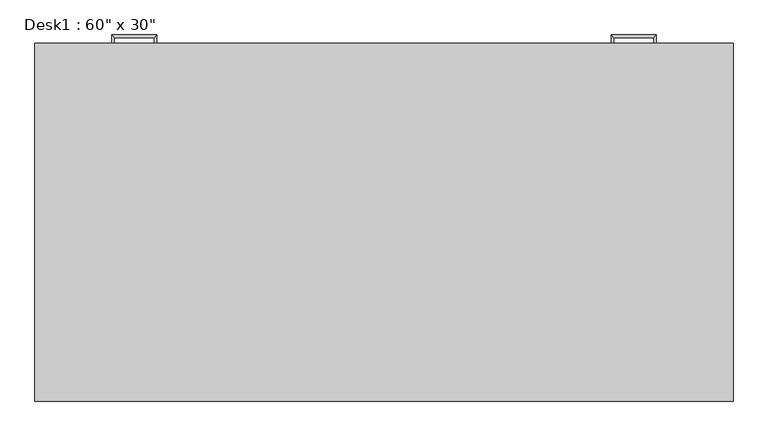
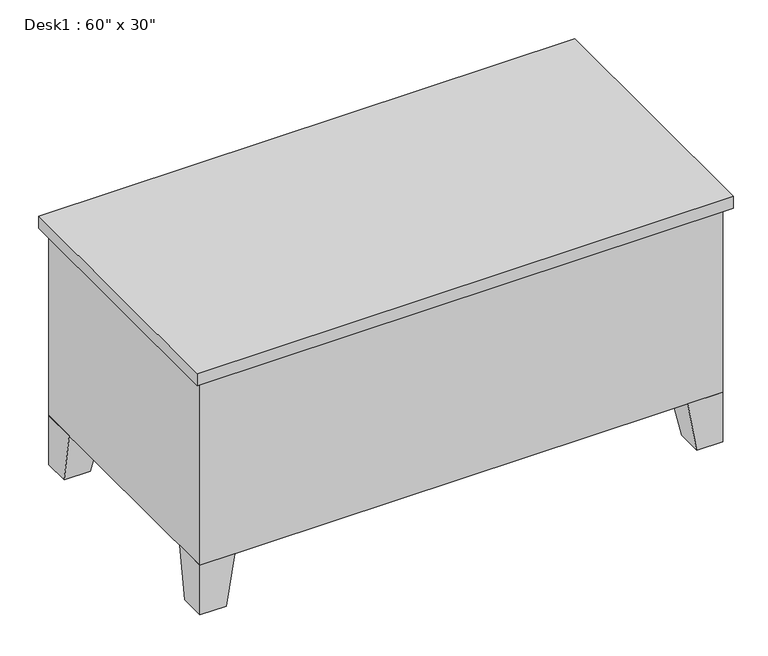
"""IFC4 building model written with IfcOpenShell, lengths in millimetres: furniture geometry."""

from ifc_helpers import new_model, si_unit, frame, origin, place, context, project, spatial, polyline, outline, extrude, faceted_brep, source, transform, mapped, element, save


def furniture_1092b3eb(model_context):
    return source(origin(), model_context, "Body", "SolidModel", [
        extrude(outline(polyline([(19.05, 0.0), (19.05, 12.7), (387.35, 12.7), (387.35, 0.0), (19.05, 0.0)])), frame((0.0, 0.0, 603.25), z_axis=(0.0, 0.0, 1.0), x_axis=(1.0, 0.0, 0.0)), (0.0, 0.0, 1.0), 101.6),
        extrude(outline(polyline([(19.05, 0.0), (19.05, 12.7), (387.35, 12.7), (387.35, 0.0), (19.05, 0.0)])), frame((0.0, 0.0, 171.45), z_axis=(0.0, 0.0, 1.0), x_axis=(1.0, 0.0, 0.0)), (0.0, 0.0, 1.0), 412.75),
        extrude(outline(polyline([(1136.65, 0.0), (1136.65, 12.7), (1504.95, 12.7), (1504.95, 0.0), (1136.65, 0.0)])), frame((0.0, 0.0, 603.25), z_axis=(0.0, 0.0, 1.0), x_axis=(1.0, 0.0, 0.0)), (0.0, 0.0, 1.0), 101.6),
        extrude(outline(polyline([(1136.65, 0.0), (1136.65, 12.7), (1504.95, 12.7), (1504.95, 0.0), (1136.65, 0.0)])), frame((0.0, 0.0, 171.45), z_axis=(0.0, 0.0, 1.0), x_axis=(1.0, 0.0, 0.0)), (0.0, 0.0, 1.0), 171.45),
        extrude(outline(polyline([(1136.65, 0.0), (1136.65, 12.7), (1504.95, 12.7), (1504.95, 0.0), (1136.65, 0.0)])), frame((0.0, 0.0, 482.6), z_axis=(0.0, 0.0, 1.0), x_axis=(1.0, 0.0, 0.0)), (0.0, 0.0, 1.0), 101.6),
        extrude(outline(polyline([(1136.65, 0.0), (1136.65, 12.7), (1504.95, 12.7), (1504.95, 0.0), (1136.65, 0.0)])), frame((0.0, 0.0, 361.95), z_axis=(0.0, 0.0, 1.0), x_axis=(1.0, 0.0, 0.0)), (0.0, 0.0, 1.0), 101.6),
        faceted_brep([(101.6, 0.0, 152.4), (0.0, 0.0, 152.4), (0.0, -101.6, 152.4), (101.6, -101.6, 152.4), (76.2, 0.0, 0.0), (76.2, -76.2, 0.0), (0.0, -76.2, 0.0), (0.0, 0.0, 0.0)], [[[0, 1, 2, 3]], [[4, 5, 6, 7]], [[4, 0, 3, 5]], [[5, 3, 2, 6]], [[6, 2, 1, 7]], [[7, 1, 0, 4]]]),
        faceted_brep([(101.6, -762.0, 152.4), (101.6, -660.4, 152.4), (0.0, -660.4, 152.4), (0.0, -762.0, 152.4), (76.2, -762.0, 0.0), (0.0, -762.0, 0.0), (0.0, -685.8, 0.0), (76.2, -685.8, 0.0)], [[[0, 1, 2, 3]], [[4, 5, 6, 7]], [[4, 0, 3, 5]], [[5, 3, 2, 6]], [[6, 2, 1, 7]], [[7, 1, 0, 4]]]),
        faceted_brep([(1422.4, -762.0, 152.4), (1524.0, -762.0, 152.4), (1524.0, -660.4, 152.4), (1422.4, -660.4, 152.4), (1447.8, -762.0, 0.0), (1447.8, -685.8, 0.0), (1524.0, -685.8, 0.0), (1524.0, -762.0, 0.0)], [[[0, 1, 2, 3]], [[4, 5, 6, 7]], [[4, 0, 3, 5]], [[5, 3, 2, 6]], [[6, 2, 1, 7]], [[7, 1, 0, 4]]]),
        faceted_brep([(1422.4, 0.0, 152.4), (1422.4, -101.6, 152.4), (1524.0, -101.6, 152.4), (1524.0, 0.0, 152.4), (1447.8, 0.0, 0.0), (1524.0, 0.0, 0.0), (1524.0, -76.2, 0.0), (1447.8, -76.2, 0.0)], [[[0, 1, 2, 3]], [[4, 5, 6, 7]], [[4, 0, 3, 5]], [[5, 3, 2, 6]], [[6, 2, 1, 7]], [[7, 1, 0, 4]]]),
        extrude(outline(polyline([(-19.05, 19.05), (1543.05, 19.05), (1543.05, -781.05), (-19.05, -781.05), (-19.05, 19.05)])), frame((0.0, 0.0, 723.9), z_axis=(0.0, 0.0, 1.0), x_axis=(1.0, 0.0, 0.0)), (0.0, 0.0, 1.0), 38.1),
        extrude(outline(polyline([(1117.6, 0.0), (1524.0, 0.0), (1524.0, -762.0), (0.0, -762.0), (0.0, 0.0), (406.4, 0.0), (406.4, -635.0), (1117.6, -635.0), (1117.6, 0.0)])), frame((0.0, 0.0, 152.4), z_axis=(0.0, 0.0, 1.0), x_axis=(1.0, 0.0, 0.0)), (0.0, 0.0, 1.0), 571.5),
        faceted_brep([(158.75, 12.7, 546.1), (152.4, 12.7, 546.1), (152.4, 12.7, 533.4), (158.75, 12.7, 533.4), (158.75, 31.75, 533.4), (158.75, 31.75, 546.1), (152.4, 38.1, 533.4), (152.4, 38.1, 546.1), (247.65, 31.75, 533.4), (247.65, 31.75, 546.1), (254.0, 38.1, 533.4), (254.0, 38.1, 546.1), (247.65, 12.7, 546.1), (247.65, 12.7, 533.4), (254.0, 12.7, 533.4), (254.0, 12.7, 546.1)], [[[0, 1, 2, 3]], [[3, 4, 5, 0]], [[2, 6, 4, 3]], [[1, 7, 6, 2]], [[0, 5, 7, 1]], [[4, 8, 9, 5]], [[6, 10, 8, 4]], [[7, 11, 10, 6]], [[5, 9, 11, 7]], [[12, 13, 14, 15]], [[8, 13, 12, 9]], [[10, 14, 13, 8]], [[11, 15, 14, 10]], [[9, 12, 15, 11]]]),
        faceted_brep([(158.75, 12.7, 666.75), (152.4, 12.7, 666.75), (152.4, 12.7, 654.05), (158.75, 12.7, 654.05), (158.75, 31.75, 654.05), (158.75, 31.75, 666.75), (152.4, 38.1, 654.05), (152.4, 38.1, 666.75), (247.65, 31.75, 654.05), (247.65, 31.75, 666.75), (254.0, 38.1, 654.05), (254.0, 38.1, 666.75), (247.65, 12.7, 666.75), (247.65, 12.7, 654.05), (254.0, 12.7, 654.05), (254.0, 12.7, 666.75)], [[[0, 1, 2, 3]], [[3, 4, 5, 0]], [[2, 6, 4, 3]], [[1, 7, 6, 2]], [[0, 5, 7, 1]], [[4, 8, 9, 5]], [[6, 10, 8, 4]], [[7, 11, 10, 6]], [[5, 9, 11, 7]], [[12, 13, 14, 15]], [[8, 13, 12, 9]], [[10, 14, 13, 8]], [[11, 15, 14, 10]], [[9, 12, 15, 11]]]),
        faceted_brep([(1365.25, 12.7, 304.8), (1365.25, 12.7, 292.1), (1371.6, 12.7, 292.1), (1371.6, 12.7, 304.8), (1371.6, 38.1, 304.8), (1365.25, 31.75, 304.8), (1371.6, 38.1, 292.1), (1365.25, 31.75, 292.1), (1270.0, 38.1, 304.8), (1276.35, 31.75, 304.8), (1270.0, 38.1, 292.1), (1276.35, 31.75, 292.1), (1276.35, 12.7, 304.8), (1270.0, 12.7, 304.8), (1270.0, 12.7, 292.1), (1276.35, 12.7, 292.1)], [[[0, 1, 2, 3]], [[3, 4, 5, 0]], [[2, 6, 4, 3]], [[1, 7, 6, 2]], [[0, 5, 7, 1]], [[4, 8, 9, 5]], [[6, 10, 8, 4]], [[7, 11, 10, 6]], [[5, 9, 11, 7]], [[12, 13, 14, 15]], [[8, 13, 12, 9]], [[10, 14, 13, 8]], [[11, 15, 14, 10]], [[9, 12, 15, 11]]]),
        faceted_brep([(1365.25, 12.7, 425.45), (1365.25, 12.7, 412.75), (1371.6, 12.7, 412.75), (1371.6, 12.7, 425.45), (1371.6, 38.1, 425.45), (1365.25, 31.75, 425.45), (1371.6, 38.1, 412.75), (1365.25, 31.75, 412.75), (1270.0, 38.1, 425.45), (1276.35, 31.75, 425.45), (1270.0, 38.1, 412.75), (1276.35, 31.75, 412.75), (1276.35, 12.7, 425.45), (1270.0, 12.7, 425.45), (1270.0, 12.7, 412.75), (1276.35, 12.7, 412.75)], [[[0, 1, 2, 3]], [[3, 4, 5, 0]], [[2, 6, 4, 3]], [[1, 7, 6, 2]], [[0, 5, 7, 1]], [[4, 8, 9, 5]], [[6, 10, 8, 4]], [[7, 11, 10, 6]], [[5, 9, 11, 7]], [[12, 13, 14, 15]], [[8, 13, 12, 9]], [[10, 14, 13, 8]], [[11, 15, 14, 10]], [[9, 12, 15, 11]]]),
        faceted_brep([(1365.25, 12.7, 546.1), (1365.25, 12.7, 533.4), (1371.6, 12.7, 533.4), (1371.6, 12.7, 546.1), (1371.6, 38.1, 546.1), (1365.25, 31.75, 546.1), (1371.6, 38.1, 533.4), (1365.25, 31.75, 533.4), (1270.0, 38.1, 546.1), (1276.35, 31.75, 546.1), (1270.0, 38.1, 533.4), (1276.35, 31.75, 533.4), (1276.35, 12.7, 546.1), (1270.0, 12.7, 546.1), (1270.0, 12.7, 533.4), (1276.35, 12.7, 533.4)], [[[0, 1, 2, 3]], [[3, 4, 5, 0]], [[2, 6, 4, 3]], [[1, 7, 6, 2]], [[0, 5, 7, 1]], [[4, 8, 9, 5]], [[6, 10, 8, 4]], [[7, 11, 10, 6]], [[5, 9, 11, 7]], [[12, 13, 14, 15]], [[8, 13, 12, 9]], [[10, 14, 13, 8]], [[11, 15, 14, 10]], [[9, 12, 15, 11]]]),
        faceted_brep([(1365.25, 12.7, 666.75), (1365.25, 12.7, 654.05), (1371.6, 12.7, 654.05), (1371.6, 12.7, 666.75), (1371.6, 38.1, 666.75), (1365.25, 31.75, 666.75), (1371.6, 38.1, 654.05), (1365.25, 31.75, 654.05), (1270.0, 38.1, 666.75), (1276.35, 31.75, 666.75), (1270.0, 38.1, 654.05), (1276.35, 31.75, 654.05), (1276.35, 12.7, 666.75), (1270.0, 12.7, 666.75), (1270.0, 12.7, 654.05), (1276.35, 12.7, 654.05)], [[[0, 1, 2, 3]], [[3, 4, 5, 0]], [[2, 6, 4, 3]], [[1, 7, 6, 2]], [[0, 5, 7, 1]], [[4, 8, 9, 5]], [[6, 10, 8, 4]], [[7, 11, 10, 6]], [[5, 9, 11, 7]], [[12, 13, 14, 15]], [[8, 13, 12, 9]], [[10, 14, 13, 8]], [[11, 15, 14, 10]], [[9, 12, 15, 11]]]),
    ])


if __name__ == "__main__":
    model = new_model("IFC4")
    model_context = context("Model", 3, world=origin())
    ifc_project = project(units=[si_unit("LENGTHUNIT", "METRE", prefix="MILLI")], contexts=[model_context])
    site = spatial("IfcSite", under=ifc_project)
    building = spatial("IfcBuilding", under=site)
    placement = place(None, origin())
    furniture_shape = furniture_1092b3eb(model_context)
    element("IfcFurniture", 1, ObjectType="Desk1 : 60\" x 30\"", at=placement, inside=building, context=model_context, shape_type="MappedRepresentation", body=[
        mapped(furniture_shape, transform((0.0, 0.0, 0.0), x_axis=(1.0, 0.0, 0.0), y_axis=(0.0, 1.0, 0.0), z_axis=(0.0, 0.0, 1.0))),
    ])
    save(model, "model.ifc")

# Revit data of these elements
# Type "Desk1 : 60\" x 30\""
#   Assembly Code = "E2020200"
#   Depth = 2' - 6"
#   Height = 2' - 6"
#   Leg Height = 0' - 6"
#   Width = 5' - 0"
#   Body Material = Laminate, Ivory, Matte
#   Handle/Leg Material = Steel, Chrome Plated
#   Top Material = Cherry
#   Default Elevation = 0
# Element 1 (IfcFurniture, "Desk1 : 60\" x 30\"")
#   Materials on its faces: "Steel, Chrome Plated", "Laminate, Ivory, Matte", "Cherry"
# Materials
#   "Laminate, Ivory, Matte": class "Plastic", colour RGB 247 247 239, transparency 0, Description = "Plastic Laminate - Ivory, Matte", Cost = 0
#   "Steel, Chrome Plated": class "Metal", colour RGB 17 17 17, transparency 0, Description = "Chromiuim plated steel", Cost = 0
#   "Cherry": class "Wood", colour RGB 226 177 128, transparency 0, Description = "Prunus Serotina", Cost = 0
